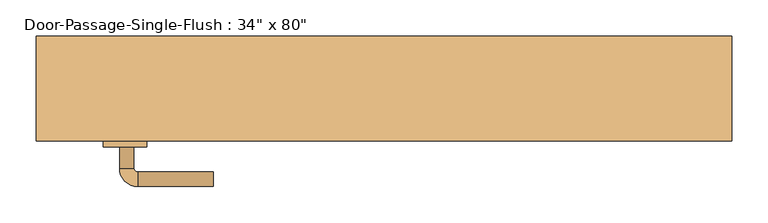
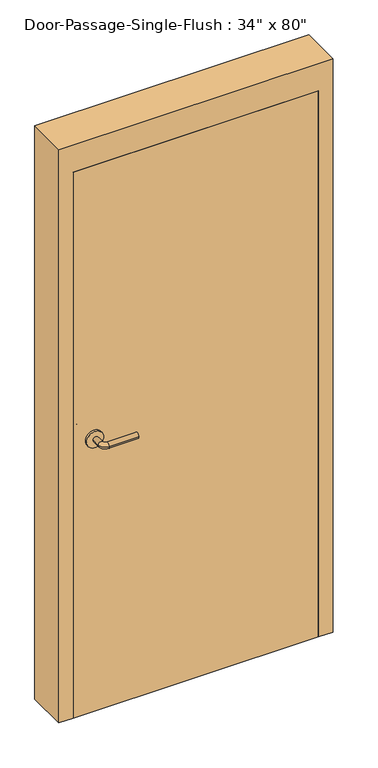
"""IFC4 building model written with IfcOpenShell, lengths in millimetres: door geometry."""

from ifc_helpers import new_model, si_unit, point, frame, frame_2d, origin, origin_with_axes, place, context, project, spatial, polyline, circle_curve, ellipse_curve, trimmed, segment, composite_curve, outline, extrude, faceted_brep, source, transform, mapped, element, save
from ifc_brep_helpers import plane_surface, cylinder_surface, revolved_surface, advanced_brep


def door_bcd5a92a(model_context):
    return source(origin(), model_context, "Body", "SolidModel", [
        advanced_brep(
        [(-366.790625, -169.8, 1016.0), (-346.790625, -169.8, 1016.0), (-366.790625, -139.8, 1016.0), (-346.790625, -139.8, 1016.0), (-341.790625, -134.8, 1016.0), (-341.790625, -114.8, 1016.0), (-236.790625, -114.8, 1016.0), (-236.790625, -134.8, 1016.0)],
        [
            (0, 1, circle_curve(frame((-356.790625, -169.8, 1016.0), z_axis=(0.0, -1.0, 0.0), x_axis=(1.0, 0.0, 0.0)), 10.0)),
            (1, 0, circle_curve(frame((-356.790625, -169.8, 1016.0), z_axis=(0.0, -1.0, 0.0), x_axis=(1.0, 0.0, 0.0)), 10.0)),
            (0, 2),
            (2, 3, circle_curve(frame((-356.790625, -139.8, 1016.0), z_axis=(0.0, -1.0, 0.0), x_axis=(1.0, 0.0, 0.0)), 10.0)),
            (3, 1),
            (3, 2, circle_curve(frame((-356.790625, -139.8, 1016.0), z_axis=(0.0, -1.0, 0.0), x_axis=(1.0, 0.0, 0.0)), 10.0)),
            (4, 3, circle_curve(frame((-341.790625, -139.8, 1016.0), z_axis=(0.0, 0.0, 1.0), x_axis=(-1.0, 0.0, 0.0)), 5.0)),
            (2, 5, circle_curve(frame((-341.790625, -139.8, 1016.0), z_axis=(0.0, 0.0, -1.0), x_axis=(-1.0, 0.0, 0.0)), 25.0)),
            (5, 4, circle_curve(frame((-341.790625, -124.8, 1016.0), z_axis=(-1.0, 0.0, 0.0), x_axis=(0.0, -1.0, 0.0)), 10.0)),
            (4, 5, circle_curve(frame((-341.790625, -124.8, 1016.0), z_axis=(-1.0, 0.0, 0.0), x_axis=(0.0, -1.0, 0.0)), 10.0)),
            (6, 7, circle_curve(frame((-236.790625, -124.8, 1016.0), z_axis=(1.0, 0.0, 0.0), x_axis=(0.0, -1.0, 0.0)), 10.0)),
            (7, 6, circle_curve(frame((-236.790625, -124.8, 1016.0), z_axis=(1.0, 0.0, 0.0), x_axis=(0.0, -1.0, 0.0)), 10.0)),
            (5, 6),
            (7, 4),
        ],
        [
            plane_surface(frame((-356.790625, -169.8, 1016.0), z_axis=(0.0, -1.0, 0.0), x_axis=(0.0, 0.0, 1.0))),
            cylinder_surface(frame((-356.790625, -169.8, 1016.0), z_axis=(0.0, -1.0, 0.0), x_axis=(1.0, 0.0, 0.0)), 10.0),
            revolved_surface(trimmed(ellipse_curve(frame((-356.790625, -139.8, 1016.0), z_axis=(0.0, -1.0, 0.0), x_axis=(1.0, 0.0, 0.0)), 10.0, 10.0), [point((-366.790625, -139.8, 1016.0))], [point((-346.790625, -139.8, 1016.0))], True, "CARTESIAN"), (-341.790625, -139.8, 1016.0), (0.0, 0.0, -1.0)),
            revolved_surface(trimmed(ellipse_curve(frame((-356.790625, -139.8, 1016.0), z_axis=(0.0, -1.0, 0.0), x_axis=(1.0, 0.0, 0.0)), 10.0, 10.0), [point((-346.790625, -139.8, 1016.0))], [point((-366.790625, -139.8, 1016.0))], True, "CARTESIAN"), (-341.790625, -139.8, 1016.0), (0.0, 0.0, -1.0)),
            plane_surface(frame((-236.790625, -124.8, 1016.0), z_axis=(1.0, 0.0, 0.0), x_axis=(0.0, 0.0, 1.0))),
            cylinder_surface(frame((-341.790625, -124.8, 1016.0), z_axis=(-1.0, 0.0, 0.0), x_axis=(0.0, -1.0, 0.0)), 10.0),
        ],
        [
            (0, [[1, 2]]),
            (1, [[-1, 3, 4, 5]]),
            (1, [[-2, -5, 6, -3]]),
            (2, [[7, -4, 8, 9]]),
            (3, [[-8, -6, -7, 10]]),
            (4, [[11, 12]]),
            (5, [[-9, 13, -12, 14]]),
            (5, [[-10, -14, -11, -13]]),
        ],
    ),
        extrude(outline(composite_curve([segment(trimmed(circle_curve(frame_2d((1016.0, -359.290625)), 30.0), [point((1016.0, -389.290625))], [point((1016.0, -329.290625))], False, "CARTESIAN"), True, "CONTINUOUS"), segment(trimmed(circle_curve(frame_2d((1016.0, -359.290625)), 30.0), [point((1016.0, -329.290625))], [point((1016.0, -389.290625))], False, "CARTESIAN"), True, "CONTINUOUS")], self_intersect=False)), frame((0.0, -177.8, 0.0), z_axis=(0.0, 1.0, 0.0), x_axis=(0.0, 0.0, 1.0)), (0.0, 0.0, 1.0), 8.0),
        advanced_brep(
        [(-366.790625, -236.6, 1016.0), (-346.790625, -236.6, 1016.0), (-346.790625, -266.6, 1016.0), (-366.790625, -266.6, 1016.0), (-341.790625, -271.6, 1016.0), (-341.790625, -291.6, 1016.0), (-236.790625, -291.6, 1016.0), (-236.790625, -271.6, 1016.0)],
        [
            (0, 1, circle_curve(frame((-356.790625, -236.6, 1016.0), z_axis=(0.0, 1.0, 0.0), x_axis=(1.0, 0.0, 0.0)), 10.0)),
            (1, 0, circle_curve(frame((-356.790625, -236.6, 1016.0), z_axis=(0.0, 1.0, 0.0), x_axis=(1.0, 0.0, 0.0)), 10.0)),
            (1, 2),
            (2, 3, circle_curve(frame((-356.790625, -266.6, 1016.0), z_axis=(0.0, 1.0, 0.0), x_axis=(1.0, 0.0, 0.0)), 10.0)),
            (3, 0),
            (3, 2, circle_curve(frame((-356.790625, -266.6, 1016.0), z_axis=(0.0, 1.0, 0.0), x_axis=(1.0, 0.0, 0.0)), 10.0)),
            (4, 5, circle_curve(frame((-341.790625, -281.6, 1016.0), z_axis=(-1.0, 0.0, 0.0), x_axis=(0.0, 1.0, 0.0)), 10.0)),
            (5, 3, circle_curve(frame((-341.790625, -266.6, 1016.0), z_axis=(0.0, 0.0, -1.0), x_axis=(-1.0, 0.0, 0.0)), 25.0)),
            (2, 4, circle_curve(frame((-341.790625, -266.6, 1016.0), z_axis=(0.0, 0.0, 1.0), x_axis=(-1.0, 0.0, 0.0)), 5.0)),
            (5, 4, circle_curve(frame((-341.790625, -281.6, 1016.0), z_axis=(-1.0, 0.0, 0.0), x_axis=(0.0, 1.0, 0.0)), 10.0)),
            (6, 7, circle_curve(frame((-236.790625, -281.6, 1016.0), z_axis=(1.0, 0.0, 0.0), x_axis=(0.0, 1.0, 0.0)), 10.0)),
            (7, 6, circle_curve(frame((-236.790625, -281.6, 1016.0), z_axis=(1.0, 0.0, 0.0), x_axis=(0.0, 1.0, 0.0)), 10.0)),
            (4, 7),
            (6, 5),
        ],
        [
            plane_surface(frame((-356.790625, -236.6, 1016.0), z_axis=(0.0, 1.0, 0.0), x_axis=(0.0, 0.0, 1.0))),
            cylinder_surface(frame((-356.790625, -236.6, 1016.0), z_axis=(0.0, 1.0, 0.0), x_axis=(1.0, 0.0, 0.0)), 10.0),
            revolved_surface(trimmed(ellipse_curve(frame((-356.790625, -266.6, 1016.0), z_axis=(0.0, -1.0, 0.0), x_axis=(1.0, 0.0, 0.0)), 10.0, 10.0), [point((-366.790625, -266.6, 1016.0))], [point((-346.790625, -266.6, 1016.0))], True, "CARTESIAN"), (-341.790625, -266.6, 1016.0), (0.0, 0.0, -1.0)),
            revolved_surface(trimmed(ellipse_curve(frame((-356.790625, -266.6, 1016.0), z_axis=(0.0, -1.0, 0.0), x_axis=(1.0, 0.0, 0.0)), 10.0, 10.0), [point((-346.790625, -266.6, 1016.0))], [point((-366.790625, -266.6, 1016.0))], True, "CARTESIAN"), (-341.790625, -266.6, 1016.0), (0.0, 0.0, -1.0)),
            plane_surface(frame((-236.790625, -281.6, 1016.0), z_axis=(1.0, 0.0, 0.0), x_axis=(0.0, 0.0, 1.0))),
            cylinder_surface(frame((-341.790625, -281.6, 1016.0), z_axis=(-1.0, 0.0, 0.0), x_axis=(0.0, 1.0, 0.0)), 10.0),
        ],
        [
            (0, [[1, 2]]),
            (1, [[3, 4, 5, -2]]),
            (1, [[-5, 6, -3, -1]]),
            (2, [[7, 8, -4, 9]]),
            (3, [[10, -9, -6, -8]]),
            (4, [[11, 12]]),
            (5, [[13, -11, 14, -7]]),
            (5, [[-14, -12, -13, -10]]),
        ],
    ),
        extrude(outline(composite_curve([segment(trimmed(circle_curve(frame_2d((1016.0, -359.290625)), 30.0), [point((1016.0, -389.290625))], [point((1016.0, -329.290625))], False, "CARTESIAN"), True, "CONTINUOUS"), segment(trimmed(circle_curve(frame_2d((1016.0, -359.290625)), 30.0), [point((1016.0, -329.290625))], [point((1016.0, -389.290625))], False, "CARTESIAN"), True, "CONTINUOUS")], self_intersect=False)), frame((0.0, -236.6, 0.0), z_axis=(0.0, 1.0, 0.0), x_axis=(0.0, 0.0, 1.0)), (0.0, 0.0, 1.0), 8.0),
        faceted_brep([(431.8, -173.0375, 0.0), (415.925, -173.0375, 0.0), (415.925, -131.7625, 0.0), (431.8, -131.7625, 0.0), (431.8, -82.55, 0.0), (482.6, -82.55, 0.0), (482.6, -228.6, 0.0), (431.8, -228.6, 0.0), (431.8, -228.6, 2032.0), (431.8, -173.0375, 2032.0), (482.6, -228.6, 2133.6), (-482.6, -228.6, 2133.6), (-482.6, -228.6, 0.0), (-431.8, -228.6, 0.0), (-431.8, -228.6, 2032.0), (482.6, -82.55, 2133.6), (431.8, -82.55, 2032.0), (-431.8, -82.55, 2032.0), (-431.8, -82.55, 0.0), (-482.6, -82.55, 0.0), (-482.6, -82.55, 2133.6), (431.8, -131.7625, 2032.0), (415.925, -131.7625, 2016.125), (-415.925, -131.7625, 2016.125), (-415.925, -131.7625, 0.0), (-431.8, -131.7625, 0.0), (-431.8, -131.7625, 2032.0), (415.925, -173.0375, 2016.125), (-431.8, -173.0375, 2032.0), (-431.8, -173.0375, 0.0), (-415.925, -173.0375, 0.0), (-415.925, -173.0375, 2016.125)], [[[0, 1, 2, 3, 4, 5, 6, 7]], [[7, 8, 9, 0]], [[6, 10, 11, 12, 13, 14, 8, 7]], [[5, 15, 10, 6]], [[4, 16, 17, 18, 19, 20, 15, 5]], [[3, 21, 16, 4]], [[2, 22, 23, 24, 25, 26, 21, 3]], [[1, 27, 22, 2]], [[0, 9, 28, 29, 30, 31, 27, 1]], [[8, 14, 28, 9]], [[16, 21, 26, 17]], [[22, 27, 31, 23]], [[12, 19, 18, 25, 24, 30, 29, 13]], [[13, 29, 28, 14]], [[11, 20, 19, 12]], [[17, 26, 25, 18]], [[23, 31, 30, 24]], [[15, 20, 11, 10]]]),
        extrude(outline(polyline([(431.8, -177.8), (431.8, -228.6), (-431.8, -228.6), (-431.8, -177.8), (431.8, -177.8)])), origin_with_axes(), (0.0, 0.0, 1.0), 2032.0),
    ])


if __name__ == "__main__":
    model = new_model("IFC4")
    model_context = context("Model", 3, world=origin())
    ifc_project = project(units=[si_unit("LENGTHUNIT", "METRE", prefix="MILLI")], contexts=[model_context])
    site = spatial("IfcSite", under=ifc_project)
    building = spatial("IfcBuilding", under=site)
    placement = place(None, origin())
    door_shape = door_bcd5a92a(model_context)
    element("IfcDoor", 1, ObjectType="Door-Passage-Single-Flush : 34\" x 80\"", at=placement, inside=building, context=model_context, shape_type="MappedRepresentation", body=[
        mapped(door_shape, transform((0.0, 0.0, 0.0), x_axis=(1.0, 0.0, 0.0), y_axis=(0.0, 1.0, 0.0), z_axis=(0.0, 0.0, 1.0))),
    ])
    save(model, "model.ifc")

# Revit data of these elements
# Type "Door-Passage-Single-Flush : 34\" x 80\""
#   Type Mark = "14"
#   Assembly Code = "C1020"
#   Analytic Construction = "Wooden"
#   Thickness = 0' - 2"
#   Thermal Resistance (R) = 2.5876 (h·ft²·°F)/BTU
#   Swing Angle [instance default] = 90.00°
#   Strike Height = 3' - 4"
#   Rough Width [instance default] = 3' - 2"
#   Rough Height [instance default] = 7' - 0"
#   Masonry Inset [instance default] = 0' - 1"
#   Masonry Frame Depth = 0' - 5 3/4"
#   MF Opening Width [instance default] = 0' - 4"
#   MF Opening Height [instance default] = 0' - 4"
#   Inset Calculate [instance default] = 0' - 4"
#   Heat Transfer Coefficient (U) = 0.3865 BTU/(h·ft²·°F)
#   Height = 6' - 8"
#   Width = 2' - 10"
#   Masonry Frame [instance default] = yes
#   Dry Wall Frame [instance default] = no
#   Panel Material = Wood - Birch
#   Door Handle Material = Aluminum
#   Frame Material = Door - Frame
#   Visual Light Transmittance = 0
#   Solar Heat Gain Coefficient = 0
#   Function = (empty or 0)
#   Wall Closure = (empty or 0)
# Element 1 (IfcDoor, "Door-Passage-Single-Flush : 34\" x 80\"")
#   Materials on its faces: "Aluminum", "Door - Frame", "Wood - Birch"
# Materials
#   "Wood - Birch": class "Unassigned", colour RGB 224 178 126, transparency 0
#   "Aluminum": class "Metal", colour RGB 244 244 244, transparency 0, Description = "Aluminum 6061", Cost = 0
#   "Door - Frame": class "Unassigned", colour RGB 118 70 51, transparency 0
